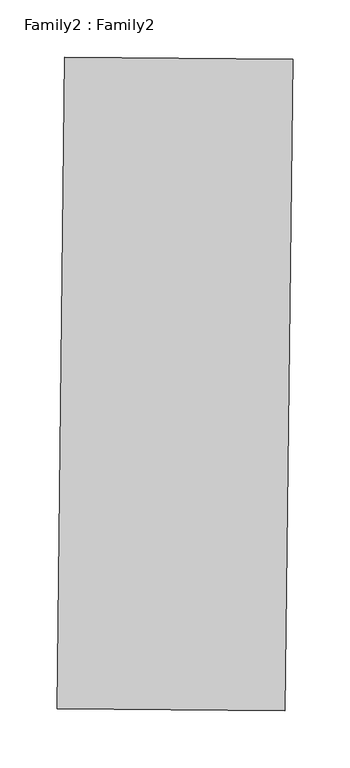
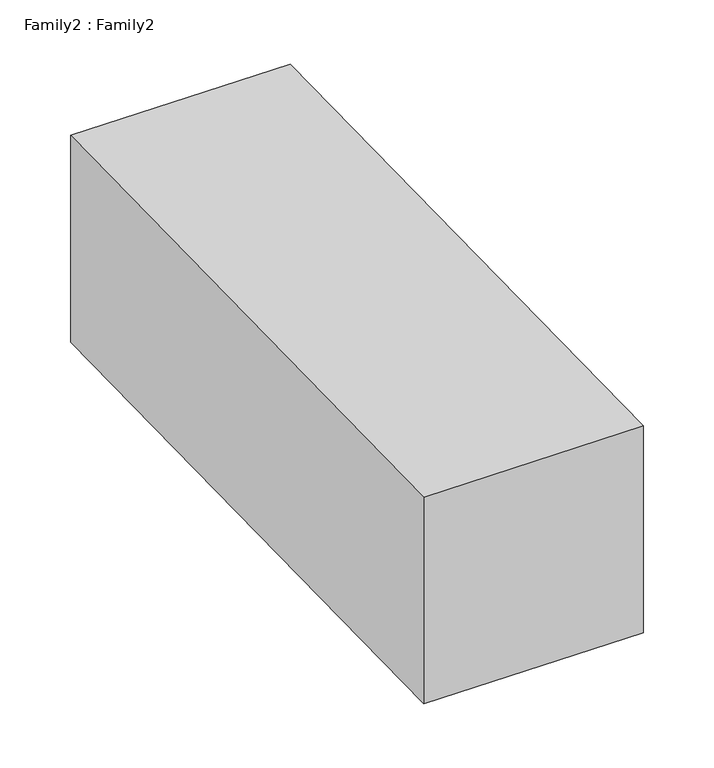
"""IFC4 building model written with IfcOpenShell, lengths in millimetres: proxy geometry, Family2 : Family2."""

import ifcopenshell
import ifcopenshell.guid

model = None  # the IFC model being written
_history = None  # IfcOwnerHistory: only IFC2X3 demands one
_inside = {}  # id of a spatial element -> (the spatial element, [elements in it])
_under = {}  # id of a project, library or spatial element -> (it, [spatial elements below it])
_declared = {}  # id of a project -> (the project, [libraries it declares])
_typed = {}  # id of a type object -> (the type object, [elements of that type])
_made_of = {}  # id of a material, layer set ... -> (it, [elements and type objects made of it])


def new_model(schema):
    """Start an empty IFC model of exactly this schema.

    Asked for "IFC4X3", IfcOpenShell would pick the latest addendum, in which some entities
    have other attributes; the version numbers below select the first issue.
    IFC2X3 requires an IfcOwnerHistory on every rooted entity: one is made here for all.
    """
    global model, _history
    if schema == "IFC4X3":
        model = ifcopenshell.file(schema_version=(4, 3, 0, 0))
    else:
        model = ifcopenshell.file(schema=schema)
    _inside.clear()
    _under.clear()
    _declared.clear()
    _typed.clear()
    _made_of.clear()
    _history = None
    if model.schema == "IFC2X3":
        org = make("IfcOrganization", Name="unknown")
        user = make(
            "IfcPersonAndOrganization",
            ThePerson=make("IfcPerson", FamilyName="unknown"),
            TheOrganization=org,
        )
        app = make(
            "IfcApplication",
            ApplicationDeveloper=org,
            Version="unknown",
            ApplicationFullName="unknown",
            ApplicationIdentifier="unknown",
        )
        _history = make(
            "IfcOwnerHistory",
            OwningUser=user,
            OwningApplication=app,
            ChangeAction="ADDED",
            CreationDate=0,
        )
    return model


def make(cls, **values):
    """One entity of the class cls with the attributes given. An attribute that is None is left unset."""
    return model.create_entity(
        cls, **{name: value for name, value in values.items() if value is not None}
    )


def rooted(cls, **values):
    """An entity with a GlobalId (a new one), such as an element, a storey or a relation."""
    return make(cls, GlobalId=ifcopenshell.guid.new(), OwnerHistory=_history, **values)


def si_unit(unit_type, name, prefix=None):
    """IfcSIUnit, for example si_unit("LENGTHUNIT", "METRE", prefix="MILLI")."""
    return make("IfcSIUnit", UnitType=unit_type, Prefix=prefix, Name=name)


def assignment(units):
    """IfcUnitAssignment: the units of a project."""
    return None if units is None else make("IfcUnitAssignment", Units=units)


def point(xyz):
    """IfcCartesianPoint."""
    return None if xyz is None else make("IfcCartesianPoint", Coordinates=xyz)


def direction(xyz):
    """IfcDirection."""
    return None if xyz is None else make("IfcDirection", DirectionRatios=xyz)


def frame(location, z_axis=None, x_axis=None):
    """IfcAxis2Placement3D, a coordinate frame: its origin and axes. An axis left out is left unset."""
    return make(
        "IfcAxis2Placement3D",
        Location=point(location),
        Axis=direction(z_axis),
        RefDirection=direction(x_axis),
    )


def origin():
    """The frame at (0, 0, 0) with its axes left unset."""
    return frame((0.0, 0.0, 0.0))


def place(relative_to, where):
    """IfcLocalPlacement: puts the frame where relative to a parent placement (None: the world)."""
    return make(
        "IfcLocalPlacement", PlacementRelTo=relative_to, RelativePlacement=where
    )


def context(
    kind, dimensions, precision=None, world=None, true_north=None, identifier=None
):
    """IfcGeometricRepresentationContext, for example the 3D "Model" context."""
    return make(
        "IfcGeometricRepresentationContext",
        ContextIdentifier=identifier,
        ContextType=kind,
        CoordinateSpaceDimension=dimensions,
        Precision=precision,
        WorldCoordinateSystem=world,
        TrueNorth=true_north,
    )


def project(units=None, contexts=None):
    """IfcProject with its units and contexts."""
    return rooted(
        "IfcProject",
        Name="project",
        RepresentationContexts=contexts,
        UnitsInContext=assignment(units),
    )


def spatial(cls, under=None, at=None, **own):
    """A site, building, storey or space (cls), placed at a placement, below another one or the project."""
    s = rooted(cls, ObjectPlacement=at, **own)
    if under is not None:
        _under.setdefault(under.id(), (under, []))[1].append(s)
    return s


def faces_of(points, faces, orient=None, outer=None):
    """IfcFace entities. A face is a list of loops; a loop is a list of indices into points, from 0.

    orient and outer hold one flag for each loop. By default every Orientation is true, the
    first loop of a face is its IfcFaceOuterBound and the others are IfcFaceBound.
    """
    made = []
    for i, loops in enumerate(faces):
        bounds = []
        for j, loop in enumerate(loops):
            is_outer = j == 0 if outer is None else outer[i][j]
            bounds.append(
                make(
                    "IfcFaceOuterBound" if is_outer else "IfcFaceBound",
                    Bound=make("IfcPolyLoop", Polygon=[points[k] for k in loop]),
                    Orientation=True if orient is None else orient[i][j],
                )
            )
        made.append(make("IfcFace", Bounds=bounds))
    return made


def faceted_brep(points, faces, orient=None, outer=None, voids=None):
    """IfcFacetedBrep: a solid bounded by flat faces; with voids (closed shells), ...WithVoids."""
    shared = [point(p) for p in points]
    hull = make("IfcClosedShell", CfsFaces=faces_of(shared, faces, orient, outer))
    if voids is None:
        return make("IfcFacetedBrep", Outer=hull)
    return make(
        "IfcFacetedBrepWithVoids",
        Outer=hull,
        Voids=[
            make(cls, CfsFaces=faces_of(shared, fs, o, b)) for cls, fs, o, b in voids
        ],
    )


def shape(context_of_items, identifier, shape_type, items):
    """IfcShapeRepresentation: the items that make up one representation, for example the "Body"."""
    return make(
        "IfcShapeRepresentation",
        ContextOfItems=context_of_items,
        RepresentationIdentifier=identifier,
        RepresentationType=shape_type,
        Items=items,
    )


def source(mapping_origin, context_of_items, identifier, shape_type, items):
    """IfcRepresentationMap: a shape defined once, which mapped items show again and again."""
    return make(
        "IfcRepresentationMap",
        MappingOrigin=mapping_origin,
        MappedRepresentation=shape(context_of_items, identifier, shape_type, items),
    )


def transform(
    local_origin,
    x_axis=None,
    y_axis=None,
    z_axis=None,
    scale=None,
    scale2=None,
    scale3=None,
    uniform=True,
):
    """IfcCartesianTransformationOperator3D, or its non-uniform kind. x_axis, y_axis, z_axis: its Axis1, 2, 3."""
    if uniform:
        return make(
            "IfcCartesianTransformationOperator3D",
            Axis1=direction(x_axis),
            Axis2=direction(y_axis),
            LocalOrigin=point(local_origin),
            Scale=scale,
            Axis3=direction(z_axis),
        )
    return make(
        "IfcCartesianTransformationOperator3DnonUniform",
        Axis1=direction(x_axis),
        Axis2=direction(y_axis),
        LocalOrigin=point(local_origin),
        Scale=scale,
        Axis3=direction(z_axis),
        Scale2=scale2,
        Scale3=scale3,
    )


def mapped(mapping_source, mapping_target):
    """IfcMappedItem: shows the shape of a source again, moved by a transform."""
    return make(
        "IfcMappedItem", MappingSource=mapping_source, MappingTarget=mapping_target
    )


def made_of(thing, what):
    """Note that an element or type object is made of a material, layer set ...; save() writes the relation."""
    if what is not None:
        _made_of.setdefault(what.id(), (what, []))[1].append(thing)
    return thing


def element(
    cls,
    number,
    at=None,
    inside=None,
    cuts=None,
    type_object=None,
    material=None,
    context=None,
    identifier="Body",
    shape_type=None,
    held_by="IfcProductDefinitionShape",
    body=None,
    shapes=None,
    **own,
):
    """One element of the class cls, such as IfcWall. Its Tag is "e" and its number.

    at: its placement. inside: the storey or other place that contains it. cuts: it is an
    opening in that element (IfcRelVoidsElement). A single representation is given by context,
    identifier, shape_type and body (its items); several are given by shapes. held_by: the class
    of the entity that holds the representations. save() writes the other relations.
    """
    e = rooted(cls, Tag="e%d" % number, ObjectPlacement=at, **own)
    if body is not None:
        shapes = [shape(context, identifier, shape_type, body)]
    if shapes is not None:
        e.Representation = make(held_by, Representations=shapes)
    if inside is not None:
        _inside.setdefault(inside.id(), (inside, []))[1].append(e)
    if cuts is not None:
        rooted(
            "IfcRelVoidsElement", RelatingBuildingElement=cuts, RelatedOpeningElement=e
        )
    if type_object is not None:
        _typed.setdefault(type_object.id(), (type_object, []))[1].append(e)
    return made_of(e, material)


def aggregate(whole, parts):
    """IfcRelAggregates: a whole, such as a stair, and the parts it consists of."""
    return rooted("IfcRelAggregates", RelatingObject=whole, RelatedObjects=parts)


def save(model, path):
    """Write the relations noted so far, then the file.

    IfcRelAggregates (storeys below a building ...), IfcRelContainedInSpatialStructure (elements
    in a storey), IfcRelDefinesByType, IfcRelAssociatesMaterial and IfcRelDeclares: one each for
    every whole, place, type object, material and project.
    """
    for whole, parts in _under.values():
        aggregate(whole, parts)
    for where, things in _inside.values():
        rooted(
            "IfcRelContainedInSpatialStructure",
            RelatedElements=things,
            RelatingStructure=where,
        )
    for kind, things in _typed.values():
        rooted("IfcRelDefinesByType", RelatedObjects=things, RelatingType=kind)
    for what, things in _made_of.values():
        rooted("IfcRelAssociatesMaterial", RelatedObjects=things, RelatingMaterial=what)
    for by, libraries in _declared.values():
        rooted("IfcRelDeclares", RelatingContext=by, RelatedDefinitions=libraries)
    model.write(path)


def family2_family2_2698309a(model_context):
    return source(origin(), model_context, "Body", "Brep", [
        faceted_brep([(-3946.9184158, -6359.5778294, 1.0945136), (-3946.9184158, -6359.5778294, 201.0945136), (-3939.9243787, -5788.0222932, 202.060409), (-3939.9243787, -5788.0222932, 2.060409), (-3746.9272258, -6361.4550421, 201.0945136), (-3739.9331888, -5789.8995058, 202.060409), (-3746.9272258, -6361.4550421, 1.0945136), (-3739.9331888, -5789.8995058, 2.060409)], [[[0, 1, 2, 3]], [[1, 4, 5, 2]], [[4, 6, 7, 5]], [[6, 0, 3, 7]], [[3, 2, 5, 7]], [[0, 6, 4, 1]]]),
    ])


if __name__ == "__main__":
    model = new_model("IFC4")
    model_context = context("Model", 3, world=origin())
    ifc_project = project(units=[si_unit("LENGTHUNIT", "METRE", prefix="MILLI")], contexts=[model_context])
    site = spatial("IfcSite", under=ifc_project)
    building = spatial("IfcBuilding", under=site)
    placement = place(None, origin())
    family2_family2_shape = family2_family2_2698309a(model_context)
    element("IfcBuildingElementProxy", 1, Name="Family2 : Family2", ObjectType="Family2 : Family2", at=placement, inside=building, context=model_context, shape_type="MappedRepresentation", body=[
        mapped(family2_family2_shape, transform((0.0, 0.0, 0.0), x_axis=(1.0, 0.0, 0.0), y_axis=(0.0, 1.0, 0.0), z_axis=(0.0, 0.0, 1.0))),
    ])
    save(model, "model.ifc")

# Revit data of these elements
# Type "Family2 : Family2"
#   Default Elevation = 0
